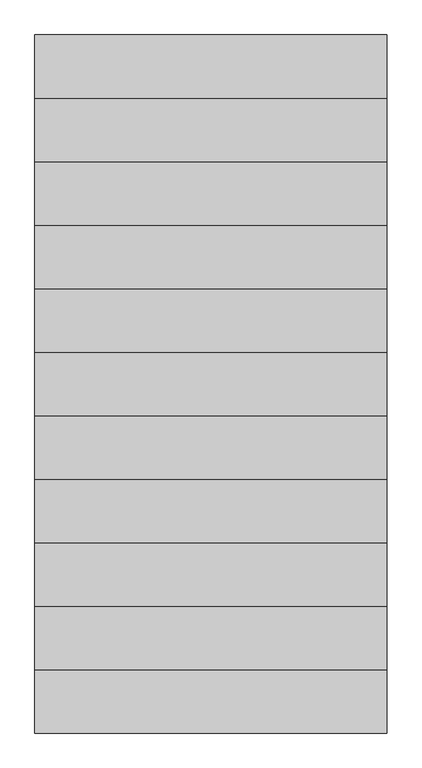
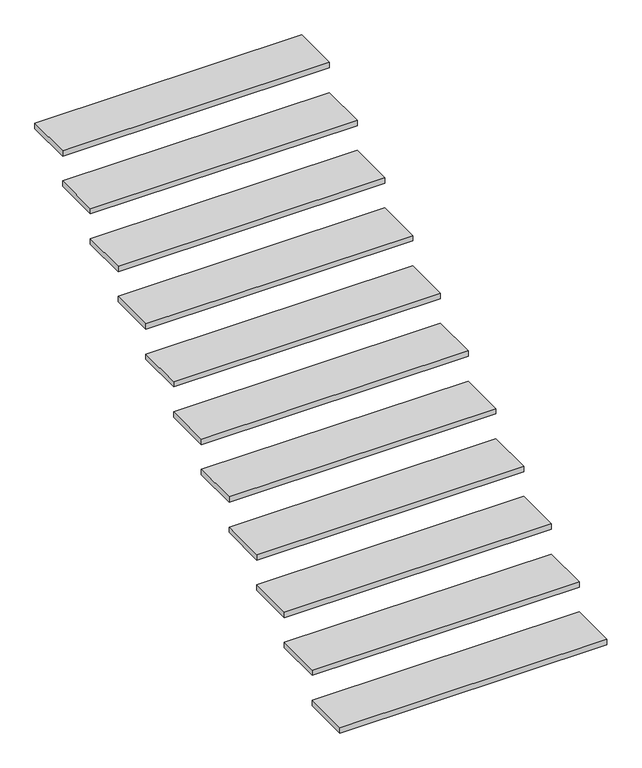
"""IFC4 building model written with IfcOpenShell, lengths in millimetres: stair flight geometry."""

from ifc_helpers import new_model, si_unit, frame, origin, place, context, project, spatial, polyline, outline, extrude, source, transform, mapped, element, save


def stair_flight_dee7d23a(model_context):
    return source(origin(), model_context, "Body", "SweptSolid", [
        extrude(outline(polyline([(17005.3403387, 2217.6066446), (18505.3403387, 2217.6066446), (18505.3403387, 1947.6066446), (17005.3403387, 1947.6066446), (17005.3403387, 2217.6066446)])), frame((0.0, 0.0, 4087.7802198), z_axis=(0.0, 0.0, 1.0), x_axis=(1.0, 0.0, 0.0)), (0.0, 0.0, 1.0), 32.0),
        extrude(outline(polyline([(17005.3403387, 2487.6066446), (18505.3403387, 2487.6066446), (18505.3403387, 2217.6066446), (17005.3403387, 2217.6066446), (17005.3403387, 2487.6066446)])), frame((0.0, 0.0, 4266.9010989), z_axis=(0.0, 0.0, 1.0), x_axis=(1.0, 0.0, 0.0)), (0.0, 0.0, 1.0), 32.0),
        extrude(outline(polyline([(17005.3403387, 2757.6066446), (18505.3403387, 2757.6066446), (18505.3403387, 2487.6066446), (17005.3403387, 2487.6066446), (17005.3403387, 2757.6066446)])), frame((0.0, 0.0, 4446.021978), z_axis=(0.0, 0.0, 1.0), x_axis=(1.0, 0.0, 0.0)), (0.0, 0.0, 1.0), 32.0),
        extrude(outline(polyline([(17005.3403387, 3027.6066446), (18505.3403387, 3027.6066446), (18505.3403387, 2757.6066446), (17005.3403387, 2757.6066446), (17005.3403387, 3027.6066446)])), frame((0.0, 0.0, 4625.1428571), z_axis=(0.0, 0.0, 1.0), x_axis=(1.0, 0.0, 0.0)), (0.0, 0.0, 1.0), 32.0),
        extrude(outline(polyline([(17005.3403387, 3297.6066446), (18505.3403387, 3297.6066446), (18505.3403387, 3027.6066446), (17005.3403387, 3027.6066446), (17005.3403387, 3297.6066446)])), frame((0.0, 0.0, 4804.2637363), z_axis=(0.0, 0.0, 1.0), x_axis=(1.0, 0.0, 0.0)), (0.0, 0.0, 1.0), 32.0),
        extrude(outline(polyline([(17005.3403387, 3567.6066446), (18505.3403387, 3567.6066446), (18505.3403387, 3297.6066446), (17005.3403387, 3297.6066446), (17005.3403387, 3567.6066446)])), frame((0.0, 0.0, 4983.3846154), z_axis=(0.0, 0.0, 1.0), x_axis=(1.0, 0.0, 0.0)), (0.0, 0.0, 1.0), 32.0),
        extrude(outline(polyline([(17005.3403387, 3837.6066446), (18505.3403387, 3837.6066446), (18505.3403387, 3567.6066446), (17005.3403387, 3567.6066446), (17005.3403387, 3837.6066446)])), frame((0.0, 0.0, 5162.5054945), z_axis=(0.0, 0.0, 1.0), x_axis=(1.0, 0.0, 0.0)), (0.0, 0.0, 1.0), 32.0),
        extrude(outline(polyline([(17005.3403387, 4107.6066446), (18505.3403387, 4107.6066446), (18505.3403387, 3837.6066446), (17005.3403387, 3837.6066446), (17005.3403387, 4107.6066446)])), frame((0.0, 0.0, 5341.6263736), z_axis=(0.0, 0.0, 1.0), x_axis=(1.0, 0.0, 0.0)), (0.0, 0.0, 1.0), 32.0),
        extrude(outline(polyline([(17005.3403387, 4377.6066446), (18505.3403387, 4377.6066446), (18505.3403387, 4107.6066446), (17005.3403387, 4107.6066446), (17005.3403387, 4377.6066446)])), frame((0.0, 0.0, 5520.7472527), z_axis=(0.0, 0.0, 1.0), x_axis=(1.0, 0.0, 0.0)), (0.0, 0.0, 1.0), 32.0),
        extrude(outline(polyline([(17005.3403387, 4647.6066446), (18505.3403387, 4647.6066446), (18505.3403387, 4377.6066446), (17005.3403387, 4377.6066446), (17005.3403387, 4647.6066446)])), frame((0.0, 0.0, 5699.8681319), z_axis=(0.0, 0.0, 1.0), x_axis=(1.0, 0.0, 0.0)), (0.0, 0.0, 1.0), 32.0),
        extrude(outline(polyline([(17005.3403387, 4917.6066446), (18505.3403387, 4917.6066446), (18505.3403387, 4647.6066446), (17005.3403387, 4647.6066446), (17005.3403387, 4917.6066446)])), frame((0.0, 0.0, 5878.989011), z_axis=(0.0, 0.0, 1.0), x_axis=(1.0, 0.0, 0.0)), (0.0, 0.0, 1.0), 32.0),
    ])


if __name__ == "__main__":
    model = new_model("IFC4")
    model_context = context("Model", 3, world=origin())
    ifc_project = project(units=[si_unit("LENGTHUNIT", "METRE", prefix="MILLI")], contexts=[model_context])
    site = spatial("IfcSite", under=ifc_project)
    building = spatial("IfcBuilding", under=site)
    placement = place(None, origin())
    stair_flight_shape = stair_flight_dee7d23a(model_context)
    element("IfcStairFlight", 1, at=placement, inside=building, context=model_context, shape_type="MappedRepresentation", body=[
        mapped(stair_flight_shape, transform((0.0, 0.0, 0.0), x_axis=(1.0, 0.0, 0.0), y_axis=(0.0, 1.0, 0.0), z_axis=(0.0, 0.0, 1.0))),
    ])
    save(model, "model.ifc")

# Revit data of these elements
# Element 1 (IfcStairFlight)
#   Materials on its faces: "철강"
# Materials
#   "철강": class "Generic", colour RGB 143 142 141, transparency 0, Description = "철골+가공조립+세우기", Cost = 0
